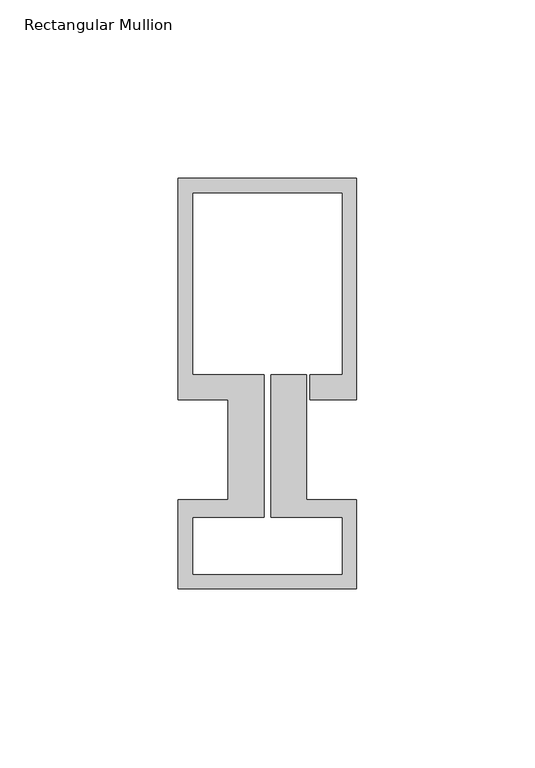
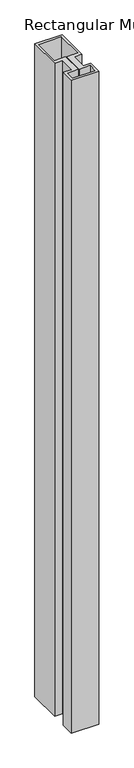
"""IFC4 building model written with IfcOpenShell, lengths in millimetres: member geometry, Rectangular Mullion : Schueco_FWS-50-HI_Tran_CovCap-20mm_Tran-55mm."""

import ifcopenshell
import ifcopenshell.guid

model = None  # the IFC model being written
_history = None  # IfcOwnerHistory: only IFC2X3 demands one
_inside = {}  # id of a spatial element -> (the spatial element, [elements in it])
_under = {}  # id of a project, library or spatial element -> (it, [spatial elements below it])
_declared = {}  # id of a project -> (the project, [libraries it declares])
_typed = {}  # id of a type object -> (the type object, [elements of that type])
_made_of = {}  # id of a material, layer set ... -> (it, [elements and type objects made of it])


def new_model(schema):
    """Start an empty IFC model of exactly this schema.

    Asked for "IFC4X3", IfcOpenShell would pick the latest addendum, in which some entities
    have other attributes; the version numbers below select the first issue.
    IFC2X3 requires an IfcOwnerHistory on every rooted entity: one is made here for all.
    """
    global model, _history
    if schema == "IFC4X3":
        model = ifcopenshell.file(schema_version=(4, 3, 0, 0))
    else:
        model = ifcopenshell.file(schema=schema)
    _inside.clear()
    _under.clear()
    _declared.clear()
    _typed.clear()
    _made_of.clear()
    _history = None
    if model.schema == "IFC2X3":
        org = make("IfcOrganization", Name="unknown")
        user = make(
            "IfcPersonAndOrganization",
            ThePerson=make("IfcPerson", FamilyName="unknown"),
            TheOrganization=org,
        )
        app = make(
            "IfcApplication",
            ApplicationDeveloper=org,
            Version="unknown",
            ApplicationFullName="unknown",
            ApplicationIdentifier="unknown",
        )
        _history = make(
            "IfcOwnerHistory",
            OwningUser=user,
            OwningApplication=app,
            ChangeAction="ADDED",
            CreationDate=0,
        )
    return model


def make(cls, **values):
    """One entity of the class cls with the attributes given. An attribute that is None is left unset."""
    return model.create_entity(
        cls, **{name: value for name, value in values.items() if value is not None}
    )


def rooted(cls, **values):
    """An entity with a GlobalId (a new one), such as an element, a storey or a relation."""
    return make(cls, GlobalId=ifcopenshell.guid.new(), OwnerHistory=_history, **values)


def si_unit(unit_type, name, prefix=None):
    """IfcSIUnit, for example si_unit("LENGTHUNIT", "METRE", prefix="MILLI")."""
    return make("IfcSIUnit", UnitType=unit_type, Prefix=prefix, Name=name)


def assignment(units):
    """IfcUnitAssignment: the units of a project."""
    return None if units is None else make("IfcUnitAssignment", Units=units)


def point(xyz):
    """IfcCartesianPoint."""
    return None if xyz is None else make("IfcCartesianPoint", Coordinates=xyz)


def direction(xyz):
    """IfcDirection."""
    return None if xyz is None else make("IfcDirection", DirectionRatios=xyz)


def frame(location, z_axis=None, x_axis=None):
    """IfcAxis2Placement3D, a coordinate frame: its origin and axes. An axis left out is left unset."""
    return make(
        "IfcAxis2Placement3D",
        Location=point(location),
        Axis=direction(z_axis),
        RefDirection=direction(x_axis),
    )


def origin():
    """The frame at (0, 0, 0) with its axes left unset."""
    return frame((0.0, 0.0, 0.0))


def place(relative_to, where):
    """IfcLocalPlacement: puts the frame where relative to a parent placement (None: the world)."""
    return make(
        "IfcLocalPlacement", PlacementRelTo=relative_to, RelativePlacement=where
    )


def context(
    kind, dimensions, precision=None, world=None, true_north=None, identifier=None
):
    """IfcGeometricRepresentationContext, for example the 3D "Model" context."""
    return make(
        "IfcGeometricRepresentationContext",
        ContextIdentifier=identifier,
        ContextType=kind,
        CoordinateSpaceDimension=dimensions,
        Precision=precision,
        WorldCoordinateSystem=world,
        TrueNorth=true_north,
    )


def project(units=None, contexts=None):
    """IfcProject with its units and contexts."""
    return rooted(
        "IfcProject",
        Name="project",
        RepresentationContexts=contexts,
        UnitsInContext=assignment(units),
    )


def spatial(cls, under=None, at=None, **own):
    """A site, building, storey or space (cls), placed at a placement, below another one or the project."""
    s = rooted(cls, ObjectPlacement=at, **own)
    if under is not None:
        _under.setdefault(under.id(), (under, []))[1].append(s)
    return s


def polyline(points):
    """IfcPolyline through the points."""
    return make("IfcPolyline", Points=[point(p) for p in points])


def outline(outer, holes=None, kind="AREA"):
    """IfcArbitraryClosedProfileDef: a profile drawn as a closed curve; with holes, ...WithVoids."""
    if holes is None:
        return make("IfcArbitraryClosedProfileDef", ProfileType=kind, OuterCurve=outer)
    return make(
        "IfcArbitraryProfileDefWithVoids",
        ProfileType=kind,
        OuterCurve=outer,
        InnerCurves=holes,
    )


def extrude(swept, where, along, depth):
    """IfcExtrudedAreaSolid: the profile swept, set in the frame where, extruded along a direction by depth."""
    return make(
        "IfcExtrudedAreaSolid",
        SweptArea=swept,
        Position=where,
        ExtrudedDirection=direction(along),
        Depth=depth,
    )


def shape(context_of_items, identifier, shape_type, items):
    """IfcShapeRepresentation: the items that make up one representation, for example the "Body"."""
    return make(
        "IfcShapeRepresentation",
        ContextOfItems=context_of_items,
        RepresentationIdentifier=identifier,
        RepresentationType=shape_type,
        Items=items,
    )


def source(mapping_origin, context_of_items, identifier, shape_type, items):
    """IfcRepresentationMap: a shape defined once, which mapped items show again and again."""
    return make(
        "IfcRepresentationMap",
        MappingOrigin=mapping_origin,
        MappedRepresentation=shape(context_of_items, identifier, shape_type, items),
    )


def transform(
    local_origin,
    x_axis=None,
    y_axis=None,
    z_axis=None,
    scale=None,
    scale2=None,
    scale3=None,
    uniform=True,
):
    """IfcCartesianTransformationOperator3D, or its non-uniform kind. x_axis, y_axis, z_axis: its Axis1, 2, 3."""
    if uniform:
        return make(
            "IfcCartesianTransformationOperator3D",
            Axis1=direction(x_axis),
            Axis2=direction(y_axis),
            LocalOrigin=point(local_origin),
            Scale=scale,
            Axis3=direction(z_axis),
        )
    return make(
        "IfcCartesianTransformationOperator3DnonUniform",
        Axis1=direction(x_axis),
        Axis2=direction(y_axis),
        LocalOrigin=point(local_origin),
        Scale=scale,
        Axis3=direction(z_axis),
        Scale2=scale2,
        Scale3=scale3,
    )


def mapped(mapping_source, mapping_target):
    """IfcMappedItem: shows the shape of a source again, moved by a transform."""
    return make(
        "IfcMappedItem", MappingSource=mapping_source, MappingTarget=mapping_target
    )


def made_of(thing, what):
    """Note that an element or type object is made of a material, layer set ...; save() writes the relation."""
    if what is not None:
        _made_of.setdefault(what.id(), (what, []))[1].append(thing)
    return thing


def element(
    cls,
    number,
    at=None,
    inside=None,
    cuts=None,
    type_object=None,
    material=None,
    context=None,
    identifier="Body",
    shape_type=None,
    held_by="IfcProductDefinitionShape",
    body=None,
    shapes=None,
    **own,
):
    """One element of the class cls, such as IfcWall. Its Tag is "e" and its number.

    at: its placement. inside: the storey or other place that contains it. cuts: it is an
    opening in that element (IfcRelVoidsElement). A single representation is given by context,
    identifier, shape_type and body (its items); several are given by shapes. held_by: the class
    of the entity that holds the representations. save() writes the other relations.
    """
    e = rooted(cls, Tag="e%d" % number, ObjectPlacement=at, **own)
    if body is not None:
        shapes = [shape(context, identifier, shape_type, body)]
    if shapes is not None:
        e.Representation = make(held_by, Representations=shapes)
    if inside is not None:
        _inside.setdefault(inside.id(), (inside, []))[1].append(e)
    if cuts is not None:
        rooted(
            "IfcRelVoidsElement", RelatingBuildingElement=cuts, RelatedOpeningElement=e
        )
    if type_object is not None:
        _typed.setdefault(type_object.id(), (type_object, []))[1].append(e)
    return made_of(e, material)


def aggregate(whole, parts):
    """IfcRelAggregates: a whole, such as a stair, and the parts it consists of."""
    return rooted("IfcRelAggregates", RelatingObject=whole, RelatedObjects=parts)


def save(model, path):
    """Write the relations noted so far, then the file.

    IfcRelAggregates (storeys below a building ...), IfcRelContainedInSpatialStructure (elements
    in a storey), IfcRelDefinesByType, IfcRelAssociatesMaterial and IfcRelDeclares: one each for
    every whole, place, type object, material and project.
    """
    for whole, parts in _under.values():
        aggregate(whole, parts)
    for where, things in _inside.values():
        rooted(
            "IfcRelContainedInSpatialStructure",
            RelatedElements=things,
            RelatingStructure=where,
        )
    for kind, things in _typed.values():
        rooted("IfcRelDefinesByType", RelatedObjects=things, RelatingType=kind)
    for what, things in _made_of.values():
        rooted("IfcRelAssociatesMaterial", RelatedObjects=things, RelatingMaterial=what)
    for by, libraries in _declared.values():
        rooted("IfcRelDeclares", RelatingContext=by, RelatedDefinitions=libraries)
    model.write(path)


def rectangular_mullion_8b143ea5(model_context):
    return source(origin(), model_context, "Body", "SweptSolid", [
        extrude(outline(polyline([(-50.0, 90.0), (0.0, 90.0), (0.0, 28.0), (-13.0, 28.0), (-13.0, 35.0), (-4.0, 35.0), (-4.0, 86.0), (-46.0, 86.0), (-46.0, 35.0), (-26.0, 35.0), (-26.0, -5.0), (-46.0, -5.0), (-46.0, -21.0), (-4.0, -21.0), (-4.0, -5.0), (-24.0, -5.0), (-24.0, 35.0), (-14.0, 35.0), (-14.0, -0.1), (0.0, -0.1), (0.0, -25.0), (-50.0, -25.0), (-50.0, -0.1), (-36.0, -0.1), (-36.0, 28.0), (-50.0, 28.0), (-50.0, 90.0)])), frame((0.0, 0.0, -1260.0), z_axis=(0.0, 0.0, 1.0), x_axis=(1.0, 0.0, 0.0)), (0.0, 0.0, 1.0), 1260.0),
    ])


if __name__ == "__main__":
    model = new_model("IFC4")
    model_context = context("Model", 3, world=origin())
    ifc_project = project(units=[si_unit("LENGTHUNIT", "METRE", prefix="MILLI")], contexts=[model_context])
    site = spatial("IfcSite", under=ifc_project)
    building = spatial("IfcBuilding", under=site)
    placement = place(None, origin())
    rectangular_mullion_shape = rectangular_mullion_8b143ea5(model_context)
    element("IfcMember", 1, ObjectType="Rectangular Mullion : Schueco_FWS-50-HI_Tran_CovCap-20mm_Tran-55mm", at=placement, inside=building, context=model_context, shape_type="MappedRepresentation", body=[
        mapped(rectangular_mullion_shape, transform((0.0, 0.0, 0.0), x_axis=(1.0, 0.0, 0.0), y_axis=(0.0, 1.0, 0.0), z_axis=(0.0, 0.0, 1.0))),
    ])
    save(model, "model.ifc")

# Revit data of these elements
# Type "Rectangular Mullion : Schueco_FWS-50-HI_Tran_CovCap-20mm_Tran-55mm"
#   Model = "FWS 50.HI"
#   Manufacturer = "Schueco International KG"
#   Type Comments = "Transom"
#   Schueco thermal insulation standard = "Highly thermally insulated"
#   Burglar resistance = "RC 3"
#   Thermal insulation = "to 0.90 W/(m²K)"
#   built-in parameter 1007322 = 0.377297 (stored number, unit not read)
#   built-in parameter 1007321 = 0.0360892 (stored number, unit not read)
#   built-in parameter 1007320 = 0.0360892 (stored number, unit not read)
# Element 1 (IfcMember, "Rectangular Mullion : Schueco_FWS-50-HI_Tran_CovCap-20mm_Tran-55mm")
#   Materials on its faces: "Alu"
# Materials
#   "Alu": class "Glas", colour RGB 140 140 140, transparency 0
